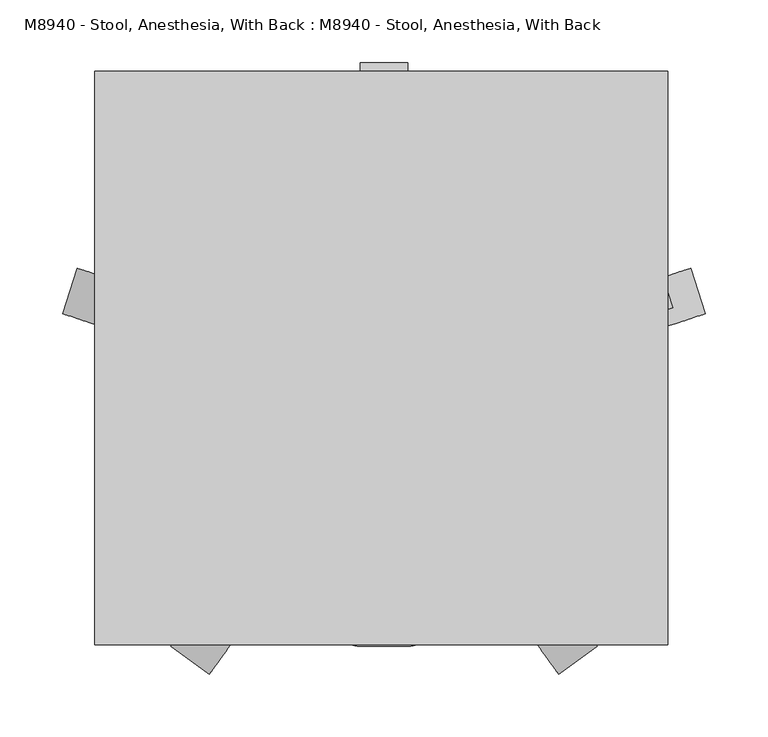
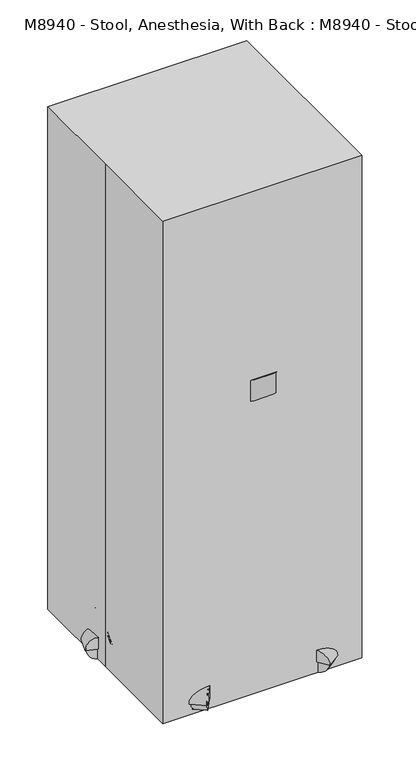
"""IFC4 building model written with IfcOpenShell, lengths in millimetres: proxy geometry, M8940 - Stool, Anesthesia, With Back : M8940 - Stool, Anesthesia, With Back."""

from ifc_helpers import new_model, si_unit, point, frame, frame_2d, origin, origin_with_axes, place, context, project, spatial, polyline, circle_curve, trimmed, segment, composite_curve, outline, extrude, source, transform, mapped, element, save


def m8940_stool_anesthesia_with_back_m8940_stool_anesthesia_with_8ebeb866(model_context):
    return source(origin(), model_context, "Body", "SweptSolid", [
        extrude(outline(polyline([(194.3763903, 810.4581371), (208.5714887, 647.7), (184.5195063, 647.7), (184.5195063, 712.4539826), (177.5948633, 811.4809912), (183.2342494, 869.54322), (199.9573639, 867.9189609), (194.3763903, 810.4581371)])), frame((-19.05, 0.0, 0.0), z_axis=(1.0, 0.0, 0.0), x_axis=(0.0, 1.0, 0.0)), (0.0, 0.0, 1.0), 40.4715924),
        extrude(outline(polyline([(212.9379653, 1088.7460454), (220.4916014, 1088.2178437), (226.7876108, 1060.1366292), (227.1133835, 1030.1498522), (216.2197136, 905.6346351), (207.041074, 851.2346071), (199.8242973, 838.5950393), (173.8183734, 840.8702628), (172.2507076, 873.7249491), (173.2697332, 883.4203304), (177.5608694, 914.372785), (182.4541996, 970.3038054), (186.0820596, 1011.7704347), (187.3514924, 1026.2801181), (188.9012405, 1074.513667), (189.8813283, 1085.716122), (212.9379653, 1088.7460454)])), frame((-209.55, 0.0, 0.0), z_axis=(1.0, 0.0, 0.0), x_axis=(0.0, 1.0, 0.0)), (0.0, 0.0, 1.0), 406.4),
        extrude(outline(composite_curve([segment(polyline([(20.4732576, 184.5195063), (20.4732576, -10.9732945)]), True, "CONTINUOUS"), segment(trimmed(circle_curve(frame_2d((1.7968221, -27.0144229)), 24.6196474), [point((20.4732576, -10.9732945))], [point((-16.8796133, -10.9732945))], True, "CARTESIAN"), True, "CONTINUOUS"), segment(polyline([(-16.8796133, -10.9732945), (-16.8796133, 184.5195063), (20.4732576, 184.5195063)]), True, "CONTINUOUS")], self_intersect=False)), frame((0.0, 0.0, 647.7), z_axis=(0.0, 0.0, 1.0), x_axis=(1.0, 0.0, 0.0)), (0.0, 0.0, 1.0), 38.1),
        extrude(outline(composite_curve([segment(trimmed(circle_curve(frame_2d((2.1703867, -27.8442581)), 203.2), [point((-201.0296133, -27.8442581))], [point((205.3703867, -27.8442581))], False, "CARTESIAN"), True, "CONTINUOUS"), segment(trimmed(circle_curve(frame_2d((2.1703867, -27.8442581)), 203.2), [point((205.3703867, -27.8442581))], [point((-201.0296133, -27.8442581))], False, "CARTESIAN"), True, "CONTINUOUS")], self_intersect=False)), frame((0.0, 0.0, 711.2), z_axis=(0.0, 0.0, 1.0), x_axis=(1.0, 0.0, 0.0)), (0.0, 0.0, 1.0), 50.8),
        extrude(outline(composite_curve([segment(trimmed(circle_curve(frame_2d((0.0, -25.7612183)), 25.7612183), [point((0.0, -51.5224365))], [point((0.0, 0.0))], False, "CARTESIAN"), True, "CONTINUOUS"), segment(trimmed(circle_curve(frame_2d((0.0, -25.7612183)), 25.7612183), [point((0.0, 0.0))], [point((0.0, -51.5224365))], False, "CARTESIAN"), True, "CONTINUOUS")], self_intersect=False)), frame((255.027118, 37.6219114, 25.7612183), z_axis=(-0.3090169943748919, 0.9510565162951716, 0.0), x_axis=(0.0, 0.0, 1.0)), (0.0, 0.0, 1.0), 31.75),
        extrude(outline(composite_curve([segment(polyline([(-57.1058785, 0.0), (-0.678315, 0.0)]), True, "CONTINUOUS"), segment(trimmed(circle_curve(frame_2d((-28.8920967, 0.0)), 28.2137817), [point((-0.678315, 0.0))], [point((-57.1058785, 0.0))], False, "CARTESIAN"), True, "CONTINUOUS")], self_intersect=False)), frame((258.9858893, 35.5698017, 25.7612183), z_axis=(-0.30901699437489194, 0.9510565162951716, 0.0), x_axis=(0.9510565162951716, 0.30901699437489194, 0.0)), (0.0, 0.0, 1.0), 38.1),
        extrude(outline(composite_curve([segment(trimmed(circle_curve(frame_2d((225.6213344, 44.7585541)), 3.5091751), [point((224.5369397, 48.0959779))], [point((226.7057291, 41.4211302))], False, "CARTESIAN"), True, "CONTINUOUS"), segment(trimmed(circle_curve(frame_2d((225.6213344, 44.7585541)), 3.5091751), [point((226.7057291, 41.4211302))], [point((224.5369397, 48.0959779))], False, "CARTESIAN"), True, "CONTINUOUS")], self_intersect=False)), frame((0.0, 0.0, 53.975), z_axis=(0.0, 0.0, 1.0), x_axis=(1.0, 0.0, 0.0)), (0.0, 0.0, 1.0), 13.49375),
        extrude(outline(polyline([(232.199718, 40.2196229), (27.5682802, -26.2691618), (23.6440039, -14.1914812), (228.2754417, 52.2973034), (232.199718, 40.2196229)])), frame((0.0, 0.0, 67.46875), z_axis=(0.0, 0.0, 1.0), x_axis=(1.0, 0.0, 0.0)), (0.0, 0.0, 1.0), 50.8),
        extrude(outline(composite_curve([segment(trimmed(circle_curve(frame_2d((0.0, -25.7612182)), 25.7612183), [point((0.0, -51.5224365))], [point((0.0, 0.0))], False, "CARTESIAN"), True, "CONTINUOUS"), segment(trimmed(circle_curve(frame_2d((0.0, -25.7612182)), 25.7612183), [point((0.0, 0.0))], [point((0.0, -51.5224365))], False, "CARTESIAN"), True, "CONTINUOUS")], self_intersect=False)), frame((142.5694409, -248.0951411, 25.7612183), z_axis=(0.8090169943749846, 0.5877852522924221, 0.0), x_axis=(0.0, 0.0, 1.0)), (0.0, 0.0, 1.0), 31.75),
        extrude(outline(composite_curve([segment(polyline([(-57.1058785, 0.0), (-0.6783151, 0.0)]), True, "CONTINUOUS"), segment(trimmed(circle_curve(frame_2d((-28.8920968, 0.0)), 28.2137817), [point((-0.6783151, 0.0))], [point((-57.1058785, 0.0))], False, "CARTESIAN"), True, "CONTINUOUS")], self_intersect=False)), frame((141.8410962, -252.4942932, 25.7612183), z_axis=(0.8090169943749845, 0.587785252292422, 0.0), x_axis=(0.587785252292422, -0.8090169943749845, 0.0)), (0.0, 0.0, 1.0), 38.1),
        extrude(outline(composite_curve([segment(trimmed(circle_curve(frame_2d((140.2699045, -217.9232351)), 3.5091751), [point((143.1088868, -215.8605938))], [point((137.4309222, -219.9858765))], False, "CARTESIAN"), True, "CONTINUOUS"), segment(trimmed(circle_curve(frame_2d((140.2699045, -217.9232351)), 3.5091751), [point((137.4309222, -219.9858765))], [point((143.1088868, -215.8605938))], False, "CARTESIAN"), True, "CONTINUOUS")], self_intersect=False)), frame((0.0, 0.0, 53.975), z_axis=(0.0, 0.0, 1.0), x_axis=(1.0, 0.0, 0.0)), (0.0, 0.0, 1.0), 13.49375),
        extrude(outline(polyline([(137.9859568, -225.5822566), (11.516773, -51.5123586), (21.7906618, -44.0479415), (148.2598455, -218.1178395), (137.9859568, -225.5822566)])), frame((0.0, 0.0, 67.46875), z_axis=(0.0, 0.0, 1.0), x_axis=(1.0, 0.0, 0.0)), (0.0, 0.0, 1.0), 50.8),
        extrude(outline(composite_curve([segment(trimmed(circle_curve(frame_2d((0.0, -25.7612183)), 25.7612183), [point((0.0, -51.5224365))], [point((0.0, 0.0))], False, "CARTESIAN"), True, "CONTINUOUS"), segment(trimmed(circle_curve(frame_2d((0.0, -25.7612183)), 25.7612183), [point((0.0, 0.0))], [point((0.0, -51.5224365))], False, "CARTESIAN"), True, "CONTINUOUS")], self_intersect=False)), frame((-138.2286675, -248.0951411, 25.7612183), z_axis=(-0.8090169943749151, 0.5877852522925178, 0.0), x_axis=(0.0, 0.0, -1.0)), (0.0, 0.0, 1.0), 31.75),
        extrude(outline(composite_curve([segment(trimmed(circle_curve(frame_2d((28.8920967, 0.0)), 28.2137817), [point((57.1058785, 0.0))], [point((0.678315, 0.0))], False, "CARTESIAN"), True, "CONTINUOUS"), segment(polyline([(0.678315, 0.0), (57.1058785, 0.0)]), True, "CONTINUOUS")], self_intersect=False)), frame((-137.5003227, -252.4942932, 25.7612183), z_axis=(-0.809016994374915, 0.5877852522925177, 0.0), x_axis=(0.5877852522925177, 0.809016994374915, 0.0)), (0.0, 0.0, 1.0), 38.1),
        extrude(outline(composite_curve([segment(trimmed(circle_curve(frame_2d((-135.9303651, -217.9223386)), 3.5091751), [point((-133.0913828, -219.98498))], [point((-138.7693474, -215.8596972))], False, "CARTESIAN"), True, "CONTINUOUS"), segment(trimmed(circle_curve(frame_2d((-135.9303651, -217.9223386)), 3.5091751), [point((-138.7693474, -215.8596972))], [point((-133.0913828, -219.98498))], False, "CARTESIAN"), True, "CONTINUOUS")], self_intersect=False)), frame((0.0, 0.0, 53.975), z_axis=(0.0, 0.0, 1.0), x_axis=(1.0, 0.0, 0.0)), (0.0, 0.0, 1.0), 13.49375),
        extrude(outline(polyline([(-143.9203061, -218.116943), (-17.4511223, -44.047045), (-7.1772336, -51.5114621), (-133.6464173, -225.58136), (-143.9203061, -218.116943)])), frame((0.0, 0.0, 67.46875), z_axis=(0.0, 0.0, 1.0), x_axis=(1.0, 0.0, 0.0)), (0.0, 0.0, 1.0), 50.8),
        extrude(outline(composite_curve([segment(trimmed(circle_curve(frame_2d((0.0, -25.7612183)), 25.7612183), [point((0.0, -51.5224365))], [point((0.0, 0.0))], False, "CARTESIAN"), True, "CONTINUOUS"), segment(trimmed(circle_curve(frame_2d((0.0, -25.7612183)), 25.7612183), [point((0.0, 0.0))], [point((0.0, -51.5224365))], False, "CARTESIAN"), True, "CONTINUOUS")], self_intersect=False)), frame((-250.6863446, 37.6219114, 25.7612183), z_axis=(0.3090169943749793, 0.9510565162951433, 0.0), x_axis=(0.0, 0.0, -1.0)), (0.0, 0.0, 1.0), 31.75),
        extrude(outline(composite_curve([segment(trimmed(circle_curve(frame_2d((28.8920968, 0.0)), 28.2137817), [point((57.1058785, 0.0))], [point((0.678315, 0.0))], False, "CARTESIAN"), True, "CONTINUOUS"), segment(polyline([(0.678315, 0.0), (57.1058785, 0.0)]), True, "CONTINUOUS")], self_intersect=False)), frame((-254.6451159, 35.5698017, 25.7612183), z_axis=(0.3090169943749793, 0.9510565162951432, 0.0), x_axis=(0.9510565162951432, -0.3090169943749793, 0.0)), (0.0, 0.0, 1.0), 38.1),
        extrude(outline(composite_curve([segment(trimmed(circle_curve(frame_2d((-221.2800896, 44.7600047)), 3.5091751), [point((-222.3644844, 41.4225809))], [point((-220.1956949, 48.0974286))], False, "CARTESIAN"), True, "CONTINUOUS"), segment(trimmed(circle_curve(frame_2d((-221.2800896, 44.7600047)), 3.5091751), [point((-220.1956949, 48.0974286))], [point((-222.3644844, 41.4225809))], False, "CARTESIAN"), True, "CONTINUOUS")], self_intersect=False)), frame((0.0, 0.0, 53.975), z_axis=(0.0, 0.0, 1.0), x_axis=(1.0, 0.0, 0.0)), (0.0, 0.0, 1.0), 13.49375),
        extrude(outline(polyline([(-223.9341969, 52.2987541), (-19.3027591, -14.1900305), (-23.2270354, -26.2677111), (-227.8584732, 40.2210735), (-223.9341969, 52.2987541)])), frame((0.0, 0.0, 67.46875), z_axis=(0.0, 0.0, 1.0), x_axis=(1.0, 0.0, 0.0)), (0.0, 0.0, 1.0), 50.8),
        extrude(outline(composite_curve([segment(trimmed(circle_curve(frame_2d((207.1057246, 25.7612183)), 25.7612183), [point((181.3445063, 25.7612183))], [point((232.8669428, 25.7612183))], False, "CARTESIAN"), True, "CONTINUOUS"), segment(trimmed(circle_curve(frame_2d((207.1057246, 25.7612183)), 25.7612183), [point((232.8669428, 25.7612183))], [point((181.3445063, 25.7612183))], False, "CARTESIAN"), True, "CONTINUOUS")], self_intersect=False)), frame((-13.7046133, 0.0, 0.0), z_axis=(1.0, 0.0, 0.0), x_axis=(0.0, 1.0, 0.0)), (0.0, 0.0, 1.0), 31.75),
        extrude(outline(composite_curve([segment(trimmed(circle_curve(frame_2d((207.1057246, 25.7612183)), 28.2137817), [point((178.8919428, 25.7612183))], [point((235.3195063, 25.7612183))], False, "CARTESIAN"), True, "CONTINUOUS"), segment(polyline([(235.3195063, 25.7612183), (178.8919428, 25.7612183)]), True, "CONTINUOUS")], self_intersect=False)), frame((-16.8796133, 0.0, 0.0), z_axis=(1.0, 0.0, 0.0), x_axis=(0.0, 1.0, 0.0)), (0.0, 0.0, 1.0), 38.1),
        extrude(outline(composite_curve([segment(trimmed(circle_curve(frame_2d((2.1711494, 207.1057246)), 3.5091751), [point((-1.3380257, 207.1057246))], [point((5.6803245, 207.1057246))], False, "CARTESIAN"), True, "CONTINUOUS"), segment(trimmed(circle_curve(frame_2d((2.1711494, 207.1057246)), 3.5091751), [point((5.6803245, 207.1057246))], [point((-1.3380257, 207.1057246))], False, "CARTESIAN"), True, "CONTINUOUS")], self_intersect=False)), frame((0.0, 0.0, 53.975), z_axis=(0.0, 0.0, 1.0), x_axis=(1.0, 0.0, 0.0)), (0.0, 0.0, 1.0), 13.49375),
        extrude(outline(polyline([(8.5207618, 211.9595323), (8.5207618, -3.2026944), (-4.178463, -3.2026944), (-4.178463, 211.9595323), (8.5207618, 211.9595323)])), frame((0.0, 0.0, 67.46875), z_axis=(0.0, 0.0, 1.0), x_axis=(1.0, 0.0, 0.0)), (0.0, 0.0, 1.0), 50.8),
        extrude(outline(composite_curve([segment(trimmed(circle_curve(frame_2d((2.1703867, -27.8442581)), 25.4466483), [point((-23.2762616, -27.8442581))], [point((27.6170351, -27.8442581))], False, "CARTESIAN"), True, "CONTINUOUS"), segment(trimmed(circle_curve(frame_2d((2.1703867, -27.8442581)), 25.4466483), [point((27.6170351, -27.8442581))], [point((-23.2762616, -27.8442581))], False, "CARTESIAN"), True, "CONTINUOUS")], self_intersect=False)), frame((0.0, 0.0, 67.46875), z_axis=(0.0, 0.0, 1.0), x_axis=(1.0, 0.0, 0.0)), (0.0, 0.0, 1.0), 643.73125),
        extrude(outline(polyline([(-228.6, 228.6), (228.6, 228.6), (228.6, -228.6), (-228.6, -228.6), (-228.6, 0.0), (-228.6, 228.6)])), origin_with_axes(), (0.0, 0.0, 1.0), 1219.2),
    ])


if __name__ == "__main__":
    model = new_model("IFC4")
    model_context = context("Model", 3, world=origin())
    ifc_project = project(units=[si_unit("LENGTHUNIT", "METRE", prefix="MILLI")], contexts=[model_context])
    site = spatial("IfcSite", under=ifc_project)
    building = spatial("IfcBuilding", under=site)
    placement = place(None, origin())
    m8940_stool_anesthesia_with_back_m8940_stool_anesthesia_with_shape = m8940_stool_anesthesia_with_back_m8940_stool_anesthesia_with_8ebeb866(model_context)
    element("IfcBuildingElementProxy", 1, Name="M8940 - Stool, Anesthesia, With Back : M8940 - Stool, Anesthesia, With Back", ObjectType="M8940 - Stool, Anesthesia, With Back : M8940 - Stool, Anesthesia, With Back", at=placement, inside=building, context=model_context, shape_type="MappedRepresentation", body=[
        mapped(m8940_stool_anesthesia_with_back_m8940_stool_anesthesia_with_shape, transform((0.0, 0.0, 0.0), x_axis=(1.0, 0.0, 0.0), y_axis=(0.0, 1.0, 0.0), z_axis=(0.0, 0.0, 1.0))),
    ])
    save(model, "model.ifc")

# Revit data of these elements
# Type "M8940 - Stool, Anesthesia, With Back : M8940 - Stool, Anesthesia, With Back"
#   Watts2 = "0"
#   Watts1 = "0"
#   Unit_Issue = "EA"
#   UTIL_6_Misc = "-"
#   UTIL_5_NonMedGas = "-"
#   UTIL_4_MiscGas = "-"
#   UTIL_3_MedGas = "-"
#   UTIL_2_Elec = "-"
#   UTIL_1_WaterDrain = "-"
#   Nomenclature = "Stool, Anesthesia, With Back"
#   NSN = "6530"
#   Location [instance default] = ""
#   JSN = "M8940"
#   Fund_Source_VA = "-"
#   Fund_Source_Navy = "-"
#   Fund_Source_Army = "-"
#   Fund_Source_AF = "-"
#   ELEC_Volts2 = "0"
#   ELEC_Volts1 = "0"
#   ELEC_Phase2 = "0"
#   ELEC_Phase1 = "0"
#   ELEC_HertzSwitch = "0"
#   ELEC_HertzDependent = "0"
#   ELEC_Hertz = "0"
#   ELEC_Amps2 = "0"
#   ELEC_Amps1 = "0"
#   DetailDescription = "Anesthesia stool with back. All stainless steel with well-curved back panel and wide conductive seat. Designed for the anesthesiologist during surgical procedures."
#   CAT_VA = "C"
#   CAT_Navy = "C"
#   CAT_IHS = "-"
#   CAT_Army = "C"
#   CAT_AF = "C"
#   BTUperhour = "0"
#   Weight_IP = 25
#   DIM_Width_IP = 1' - 6"
#   DIM_Height_IP = 4' - 0"
#   DIM_Depth_IP = 1' - 6"
# Element 1 (IfcBuildingElementProxy, "M8940 - Stool, Anesthesia, With Back : M8940 - Stool, Anesthesia, With Back")
#   Materials on its faces: "Stool metal", "Stool caster", "EquipSpace"
# Materials
#   "Stool metal": class "Unassigned", colour RGB 201 201 201, transparency 0, Comments = "Rendering appearance not upgraded "
#   "Stool caster": class "Unassigned", colour RGB 0 0 0, transparency 0, Comments = "Rendering appearance not upgraded "
#   "EquipSpace": class "Unassigned", colour RGB 221 217 195, transparency 0.5
